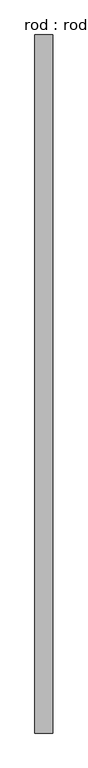
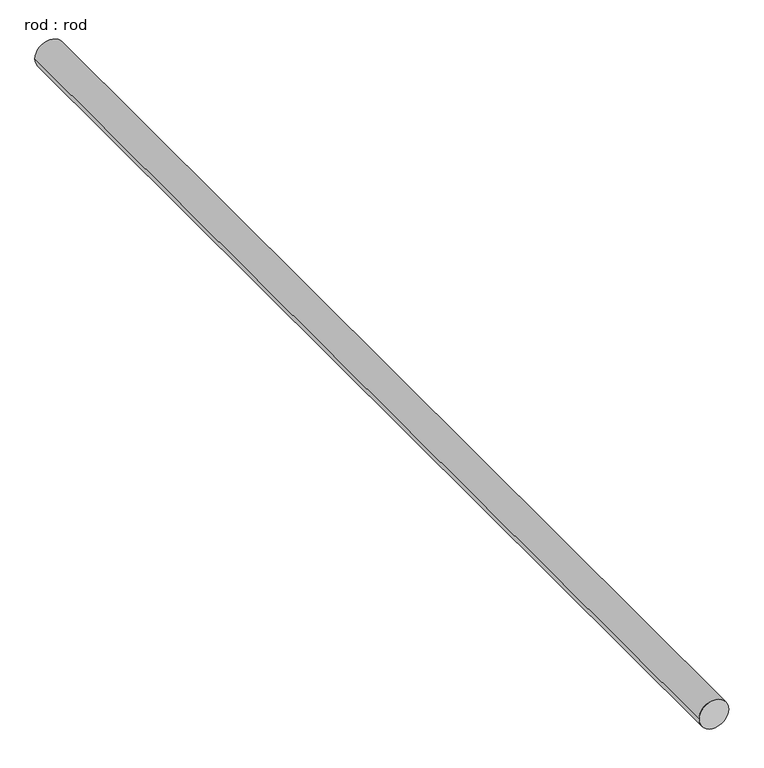
"""IFC4 building model written with IfcOpenShell, lengths in millimetres: proxy geometry, rod : rod."""

import ifcopenshell
import ifcopenshell.guid

model = None  # the IFC model being written
_history = None  # IfcOwnerHistory: only IFC2X3 demands one
_inside = {}  # id of a spatial element -> (the spatial element, [elements in it])
_under = {}  # id of a project, library or spatial element -> (it, [spatial elements below it])
_declared = {}  # id of a project -> (the project, [libraries it declares])
_typed = {}  # id of a type object -> (the type object, [elements of that type])
_made_of = {}  # id of a material, layer set ... -> (it, [elements and type objects made of it])


def new_model(schema):
    """Start an empty IFC model of exactly this schema.

    Asked for "IFC4X3", IfcOpenShell would pick the latest addendum, in which some entities
    have other attributes; the version numbers below select the first issue.
    IFC2X3 requires an IfcOwnerHistory on every rooted entity: one is made here for all.
    """
    global model, _history
    if schema == "IFC4X3":
        model = ifcopenshell.file(schema_version=(4, 3, 0, 0))
    else:
        model = ifcopenshell.file(schema=schema)
    _inside.clear()
    _under.clear()
    _declared.clear()
    _typed.clear()
    _made_of.clear()
    _history = None
    if model.schema == "IFC2X3":
        org = make("IfcOrganization", Name="unknown")
        user = make(
            "IfcPersonAndOrganization",
            ThePerson=make("IfcPerson", FamilyName="unknown"),
            TheOrganization=org,
        )
        app = make(
            "IfcApplication",
            ApplicationDeveloper=org,
            Version="unknown",
            ApplicationFullName="unknown",
            ApplicationIdentifier="unknown",
        )
        _history = make(
            "IfcOwnerHistory",
            OwningUser=user,
            OwningApplication=app,
            ChangeAction="ADDED",
            CreationDate=0,
        )
    return model


def make(cls, **values):
    """One entity of the class cls with the attributes given. An attribute that is None is left unset."""
    return model.create_entity(
        cls, **{name: value for name, value in values.items() if value is not None}
    )


def rooted(cls, **values):
    """An entity with a GlobalId (a new one), such as an element, a storey or a relation."""
    return make(cls, GlobalId=ifcopenshell.guid.new(), OwnerHistory=_history, **values)


def si_unit(unit_type, name, prefix=None):
    """IfcSIUnit, for example si_unit("LENGTHUNIT", "METRE", prefix="MILLI")."""
    return make("IfcSIUnit", UnitType=unit_type, Prefix=prefix, Name=name)


def assignment(units):
    """IfcUnitAssignment: the units of a project."""
    return None if units is None else make("IfcUnitAssignment", Units=units)


def point(xyz):
    """IfcCartesianPoint."""
    return None if xyz is None else make("IfcCartesianPoint", Coordinates=xyz)


def direction(xyz):
    """IfcDirection."""
    return None if xyz is None else make("IfcDirection", DirectionRatios=xyz)


def frame(location, z_axis=None, x_axis=None):
    """IfcAxis2Placement3D, a coordinate frame: its origin and axes. An axis left out is left unset."""
    return make(
        "IfcAxis2Placement3D",
        Location=point(location),
        Axis=direction(z_axis),
        RefDirection=direction(x_axis),
    )


def frame_2d(location, x_axis=None):
    """IfcAxis2Placement2D, a coordinate frame in the plane: its origin and x axis."""
    return make(
        "IfcAxis2Placement2D", Location=point(location), RefDirection=direction(x_axis)
    )


def origin():
    """The frame at (0, 0, 0) with its axes left unset."""
    return frame((0.0, 0.0, 0.0))


def place(relative_to, where):
    """IfcLocalPlacement: puts the frame where relative to a parent placement (None: the world)."""
    return make(
        "IfcLocalPlacement", PlacementRelTo=relative_to, RelativePlacement=where
    )


def context(
    kind, dimensions, precision=None, world=None, true_north=None, identifier=None
):
    """IfcGeometricRepresentationContext, for example the 3D "Model" context."""
    return make(
        "IfcGeometricRepresentationContext",
        ContextIdentifier=identifier,
        ContextType=kind,
        CoordinateSpaceDimension=dimensions,
        Precision=precision,
        WorldCoordinateSystem=world,
        TrueNorth=true_north,
    )


def project(units=None, contexts=None):
    """IfcProject with its units and contexts."""
    return rooted(
        "IfcProject",
        Name="project",
        RepresentationContexts=contexts,
        UnitsInContext=assignment(units),
    )


def spatial(cls, under=None, at=None, **own):
    """A site, building, storey or space (cls), placed at a placement, below another one or the project."""
    s = rooted(cls, ObjectPlacement=at, **own)
    if under is not None:
        _under.setdefault(under.id(), (under, []))[1].append(s)
    return s


def circle_curve(where, radius):
    """IfcCircle in the frame where."""
    return make("IfcCircle", Position=where, Radius=radius)


def trimmed(basis, trim1, trim2, sense, master):
    """IfcTrimmedCurve: the piece of a basis curve between two trims."""
    return make(
        "IfcTrimmedCurve",
        BasisCurve=basis,
        Trim1=trim1,
        Trim2=trim2,
        SenseAgreement=sense,
        MasterRepresentation=master,
    )


def segment(curve, same_sense, transition):
    """IfcCompositeCurveSegment."""
    return make(
        "IfcCompositeCurveSegment",
        Transition=transition,
        SameSense=same_sense,
        ParentCurve=curve,
    )


def composite_curve(segments, self_intersect=None):
    """IfcCompositeCurve: segments joined end to end."""
    return make("IfcCompositeCurve", Segments=segments, SelfIntersect=self_intersect)


def outline(outer, holes=None, kind="AREA"):
    """IfcArbitraryClosedProfileDef: a profile drawn as a closed curve; with holes, ...WithVoids."""
    if holes is None:
        return make("IfcArbitraryClosedProfileDef", ProfileType=kind, OuterCurve=outer)
    return make(
        "IfcArbitraryProfileDefWithVoids",
        ProfileType=kind,
        OuterCurve=outer,
        InnerCurves=holes,
    )


def extrude(swept, where, along, depth):
    """IfcExtrudedAreaSolid: the profile swept, set in the frame where, extruded along a direction by depth."""
    return make(
        "IfcExtrudedAreaSolid",
        SweptArea=swept,
        Position=where,
        ExtrudedDirection=direction(along),
        Depth=depth,
    )


def shape(context_of_items, identifier, shape_type, items):
    """IfcShapeRepresentation: the items that make up one representation, for example the "Body"."""
    return make(
        "IfcShapeRepresentation",
        ContextOfItems=context_of_items,
        RepresentationIdentifier=identifier,
        RepresentationType=shape_type,
        Items=items,
    )


def source(mapping_origin, context_of_items, identifier, shape_type, items):
    """IfcRepresentationMap: a shape defined once, which mapped items show again and again."""
    return make(
        "IfcRepresentationMap",
        MappingOrigin=mapping_origin,
        MappedRepresentation=shape(context_of_items, identifier, shape_type, items),
    )


def transform(
    local_origin,
    x_axis=None,
    y_axis=None,
    z_axis=None,
    scale=None,
    scale2=None,
    scale3=None,
    uniform=True,
):
    """IfcCartesianTransformationOperator3D, or its non-uniform kind. x_axis, y_axis, z_axis: its Axis1, 2, 3."""
    if uniform:
        return make(
            "IfcCartesianTransformationOperator3D",
            Axis1=direction(x_axis),
            Axis2=direction(y_axis),
            LocalOrigin=point(local_origin),
            Scale=scale,
            Axis3=direction(z_axis),
        )
    return make(
        "IfcCartesianTransformationOperator3DnonUniform",
        Axis1=direction(x_axis),
        Axis2=direction(y_axis),
        LocalOrigin=point(local_origin),
        Scale=scale,
        Axis3=direction(z_axis),
        Scale2=scale2,
        Scale3=scale3,
    )


def mapped(mapping_source, mapping_target):
    """IfcMappedItem: shows the shape of a source again, moved by a transform."""
    return make(
        "IfcMappedItem", MappingSource=mapping_source, MappingTarget=mapping_target
    )


def made_of(thing, what):
    """Note that an element or type object is made of a material, layer set ...; save() writes the relation."""
    if what is not None:
        _made_of.setdefault(what.id(), (what, []))[1].append(thing)
    return thing


def element(
    cls,
    number,
    at=None,
    inside=None,
    cuts=None,
    type_object=None,
    material=None,
    context=None,
    identifier="Body",
    shape_type=None,
    held_by="IfcProductDefinitionShape",
    body=None,
    shapes=None,
    **own,
):
    """One element of the class cls, such as IfcWall. Its Tag is "e" and its number.

    at: its placement. inside: the storey or other place that contains it. cuts: it is an
    opening in that element (IfcRelVoidsElement). A single representation is given by context,
    identifier, shape_type and body (its items); several are given by shapes. held_by: the class
    of the entity that holds the representations. save() writes the other relations.
    """
    e = rooted(cls, Tag="e%d" % number, ObjectPlacement=at, **own)
    if body is not None:
        shapes = [shape(context, identifier, shape_type, body)]
    if shapes is not None:
        e.Representation = make(held_by, Representations=shapes)
    if inside is not None:
        _inside.setdefault(inside.id(), (inside, []))[1].append(e)
    if cuts is not None:
        rooted(
            "IfcRelVoidsElement", RelatingBuildingElement=cuts, RelatedOpeningElement=e
        )
    if type_object is not None:
        _typed.setdefault(type_object.id(), (type_object, []))[1].append(e)
    return made_of(e, material)


def aggregate(whole, parts):
    """IfcRelAggregates: a whole, such as a stair, and the parts it consists of."""
    return rooted("IfcRelAggregates", RelatingObject=whole, RelatedObjects=parts)


def save(model, path):
    """Write the relations noted so far, then the file.

    IfcRelAggregates (storeys below a building ...), IfcRelContainedInSpatialStructure (elements
    in a storey), IfcRelDefinesByType, IfcRelAssociatesMaterial and IfcRelDeclares: one each for
    every whole, place, type object, material and project.
    """
    for whole, parts in _under.values():
        aggregate(whole, parts)
    for where, things in _inside.values():
        rooted(
            "IfcRelContainedInSpatialStructure",
            RelatedElements=things,
            RelatingStructure=where,
        )
    for kind, things in _typed.values():
        rooted("IfcRelDefinesByType", RelatedObjects=things, RelatingType=kind)
    for what, things in _made_of.values():
        rooted("IfcRelAssociatesMaterial", RelatedObjects=things, RelatingMaterial=what)
    for by, libraries in _declared.values():
        rooted("IfcRelDeclares", RelatingContext=by, RelatedDefinitions=libraries)
    model.write(path)


def rod_rod_87444a29(model_context):
    return source(origin(), model_context, "Body", "SweptSolid", [
        extrude(outline(composite_curve([segment(trimmed(circle_curve(frame_2d((0.0108462, 0.0)), 200.0), [point((0.0108462, 200.0))], [point((0.0108462, -200.0))], False, "CARTESIAN"), True, "CONTINUOUS"), segment(trimmed(circle_curve(frame_2d((0.0108462, 0.0)), 200.0), [point((0.0108462, -200.0))], [point((0.0108462, 200.0))], False, "CARTESIAN"), True, "CONTINUOUS")], self_intersect=False)), frame((0.0, -3658.3852283, 0.0), z_axis=(0.0, 1.0, 0.0), x_axis=(0.0, 0.0, 1.0)), (0.0, 0.0, 1.0), 15502.2276872),
    ])


if __name__ == "__main__":
    model = new_model("IFC4")
    model_context = context("Model", 3, world=origin())
    ifc_project = project(units=[si_unit("LENGTHUNIT", "METRE", prefix="MILLI")], contexts=[model_context])
    site = spatial("IfcSite", under=ifc_project)
    building = spatial("IfcBuilding", under=site)
    placement = place(None, origin())
    rod_rod_shape = rod_rod_87444a29(model_context)
    element("IfcBuildingElementProxy", 1, Name="rod : rod", ObjectType="rod : rod", at=placement, inside=building, context=model_context, shape_type="MappedRepresentation", body=[
        mapped(rod_rod_shape, transform((0.0, 0.0, 0.0), x_axis=(1.0, 0.0, 0.0), y_axis=(0.0, 1.0, 0.0), z_axis=(0.0, 0.0, 1.0))),
    ])
    save(model, "model.ifc")

# Revit data of these elements
# Type "rod : rod"
#   Default Elevation = 0
